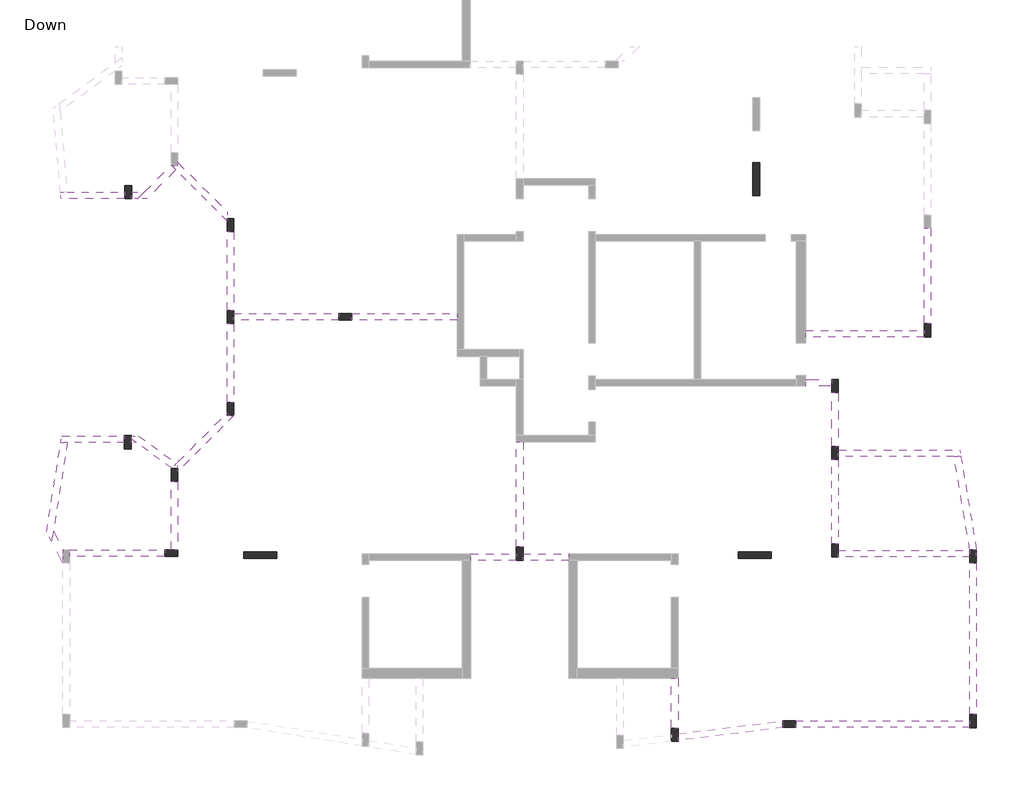
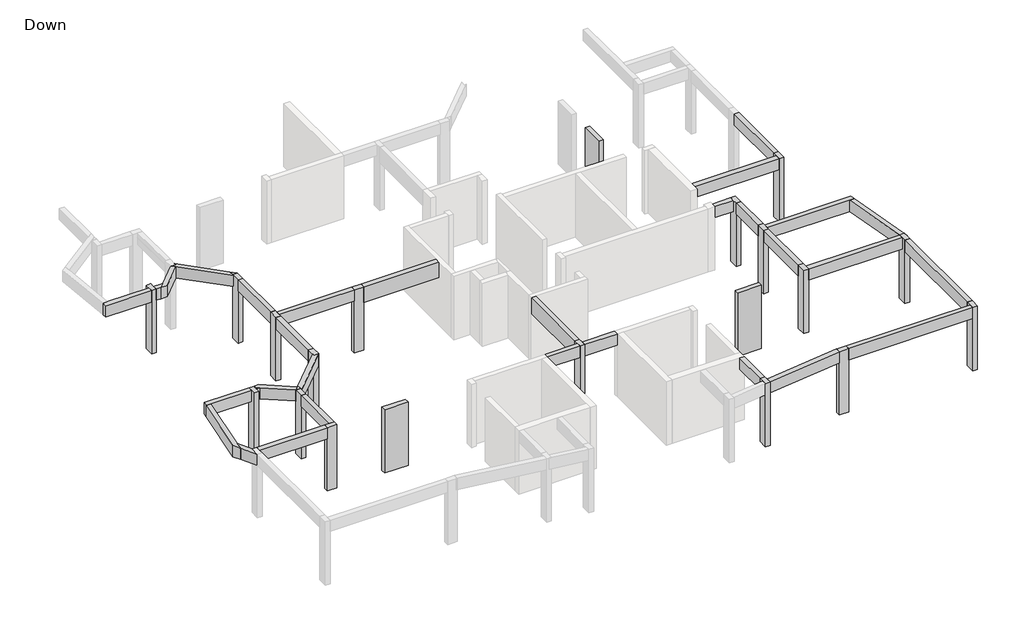
# One storey, part 2 of 3: 31 beams, 20 columns.
# Revit data of these elements (continued)
# Element 41 (IfcColumn, "Concrete Rectengular Column : 20/40") (continued)
#   SOFiSTiK_AMG_Scheduled = yes
#   SOFiSTiK_AMG_Adjusted = yes
#   Structural Material = Concrete
#   Phase Created = New Construction
#   Materials on its faces: "Concrete"
# Element 42 (IfcColumn, "Concrete Rectengular Column : 20/40")
#   Comments = ""
#   Mark = "C28"
#   SOFiSTiK_AMG_Comments = ""
#   SOFiSTiK_AMG_Scheduled = yes
#   SOFiSTiK_AMG_Adjusted = yes
#   Structural Material = Concrete
#   Phase Created = New Construction
#   Materials on its faces: "Concrete"
# Element 43 (IfcColumn, "Concrete Rectengular Column : 20/40")
#   Comments = ""
#   Mark = "C30"
#   SOFiSTiK_AMG_Comments = ""
#   SOFiSTiK_AMG_Scheduled = yes
#   SOFiSTiK_AMG_Adjusted = yes
#   Structural Material = Concrete
#   Phase Created = New Construction
#   Materials on its faces: "Concrete"
# Element 44 (IfcColumn, "Concrete Rectengular Column : 20/40")
#   Comments = ""
#   Mark = "C31"
#   SOFiSTiK_AMG_Comments = ""
#   SOFiSTiK_AMG_Scheduled = yes
#   SOFiSTiK_AMG_Adjusted = yes
#   Structural Material = Concrete
#   Phase Created = New Construction
#   Materials on its faces: "Concrete"
# Element 45 (IfcColumn, "Concrete Rectengular Column : 20/40")
#   Comments = ""
#   Mark = "C32"
#   SOFiSTiK_AMG_Comments = ""
#   SOFiSTiK_AMG_Scheduled = yes
#   SOFiSTiK_AMG_Adjusted = yes
#   Structural Material = Concrete
#   Phase Created = New Construction
#   Materials on its faces: "Concrete"
# Element 46 (IfcColumn, "Concrete Rectengular Column : 20/40")
#   Comments = ""
#   Mark = "C33"
#   SOFiSTiK_AMG_Comments = ""
#   SOFiSTiK_AMG_Scheduled = yes
#   SOFiSTiK_AMG_Adjusted = yes
#   Structural Material = Concrete
#   Phase Created = New Construction
#   Materials on its faces: "Concrete"
# Element 47 (IfcColumn, "Concrete Rectengular Column : 20/40")
#   Comments = ""
#   Mark = "C34"
#   SOFiSTiK_AMG_Comments = ""
#   SOFiSTiK_AMG_Scheduled = yes
#   SOFiSTiK_AMG_Adjusted = yes
#   Structural Material = Concrete
#   Phase Created = New Construction
#   Materials on its faces: "Concrete"
# Element 48 (IfcColumn, "Concrete Rectengular Column : 20/40")
#   Comments = ""
#   Mark = "C35"
#   SOFiSTiK_AMG_Comments = ""
#   SOFiSTiK_AMG_Scheduled = yes
#   SOFiSTiK_AMG_Adjusted = yes
#   Structural Material = Concrete
#   Phase Created = New Construction
#   Materials on its faces: "Concrete"
# Element 49 (IfcColumn, "Concrete Rectengular Column : 20/40")
#   Comments = ""
#   Mark = "C36"
#   SOFiSTiK_AMG_Comments = ""
#   SOFiSTiK_AMG_Scheduled = yes
#   SOFiSTiK_AMG_Adjusted = yes
#   Structural Material = Concrete
#   Phase Created = New Construction
#   Materials on its faces: "Concrete"
# Element 50 (IfcColumn, "Concrete Rectengular Column : 20/40")
#   Comments = ""
#   Mark = "C37"
#   SOFiSTiK_AMG_Comments = ""
#   SOFiSTiK_AMG_Scheduled = yes
#   SOFiSTiK_AMG_Adjusted = yes
#   Structural Material = Concrete
#   Phase Created = New Construction
#   Materials on its faces: "Concrete"
# Element 51 (IfcColumn, "Concrete Rectengular Column : 20/40")
#   Comments = ""
#   Mark = "C39"
#   SOFiSTiK_AMG_Comments = ""
#   SOFiSTiK_AMG_Scheduled = yes
#   SOFiSTiK_AMG_Adjusted = yes
#   Structural Material = Concrete
#   Phase Created = New Construction
#   Materials on its faces: "Concrete"
# Materials
#   "Concrete": class "Concrete", colour RGB 192 192 192, transparency 0, Keynote = "01000", Description = "Cast-in-place concrete", Cost = 0
